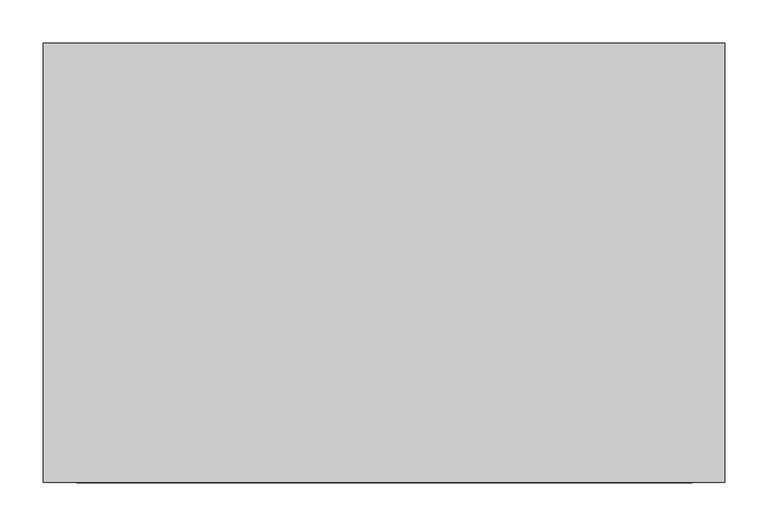
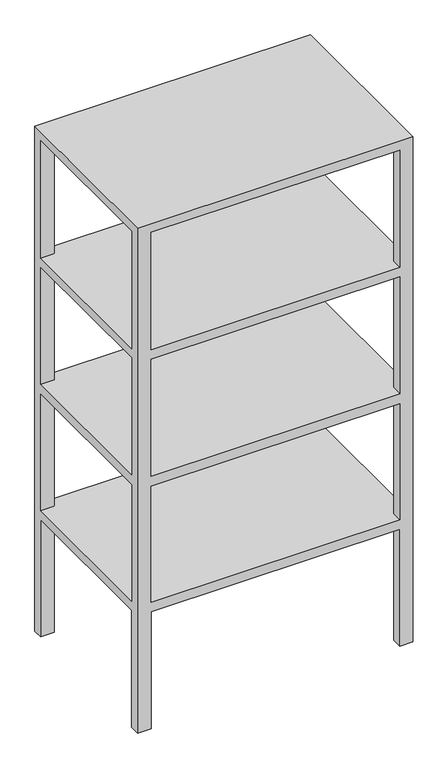
"""IFC4 building model written with IfcOpenShell, lengths in millimetres: furniture geometry, Preserved mushrrom shelf : Preserved mushrrom shelf."""

from ifc_helpers import new_model, si_unit, origin, place, context, project, spatial, faceted_brep, source, transform, mapped, element, save


def furniture_d8989670(model_context):
    return source(origin(), model_context, "Body", "Brep", [
        faceted_brep([(10489.488508, 3379.4615366, 1524.0), (9702.088508, 3379.4615366, 1524.0), (9702.088508, 2871.4615366, 1524.0), (10489.488508, 2871.4615366, 1524.0), (10489.488508, 2900.385331, 0.0), (10489.488508, 2871.4615366, 0.0), (10452.1087778, 2871.4615366, 0.0), (10452.1087778, 2900.385331, 0.0), (10489.488508, 3379.4615366, 0.0), (10489.488508, 3350.4392676, 0.0), (10452.1087778, 3350.4392676, 0.0), (10452.1087778, 3379.4615366, 0.0), (9740.9087778, 2871.4615366, 0.0), (9702.088508, 2871.4615366, 0.0), (9702.088508, 2900.385331, 0.0), (9740.9087778, 2900.385331, 0.0), (9702.088508, 3350.4392676, 0.0), (9702.088508, 3379.4615366, 0.0), (9740.9087778, 3379.4615366, 0.0), (9740.9087778, 3350.4392676, 0.0), (10452.1087778, 3379.4615366, 353.3332002), (9740.9087778, 3379.4615366, 353.3332002), (10452.1087778, 3379.4615366, 1497.6781444), (9740.9087778, 3379.4615366, 1497.6781444), (9740.9087778, 3379.4615366, 1143.0), (10452.1087778, 3379.4615366, 1143.0), (10452.1087778, 3379.4615366, 1114.8196695), (9740.9087778, 3379.4615366, 1114.8196695), (9740.9087778, 3379.4615366, 762.0), (10452.1087778, 3379.4615366, 762.0), (10452.1087778, 3379.4615366, 731.9611947), (9740.9087778, 3379.4615366, 731.9611947), (9740.9087778, 3379.4615366, 381.0), (10452.1087778, 3379.4615366, 381.0), (9702.088508, 3350.4392676, 353.3332002), (9702.088508, 2900.385331, 353.3332002), (9702.088508, 3350.8671384, 1497.6781444), (9702.088508, 2900.385331, 1497.6781444), (9702.088508, 2900.385331, 1143.0), (9702.088508, 3350.8671384, 1143.0), (9702.088508, 3350.4392676, 1114.8196695), (9702.088508, 2900.385331, 1114.8196695), (9702.088508, 2900.385331, 762.0), (9702.088508, 3350.4392676, 762.0), (9702.088508, 3350.4392676, 731.9611947), (9702.088508, 2900.385331, 731.9611947), (9702.088508, 2900.385331, 381.0), (9702.088508, 3350.4392676, 381.0), (9740.9087778, 2871.4615366, 353.3332002), (10452.1087778, 2871.4615366, 353.3332002), (9740.9087778, 2871.4615366, 1497.6781444), (10452.1087778, 2871.4615366, 1497.6781444), (10452.1087778, 2871.4615366, 1143.0), (9740.9087778, 2871.4615366, 1143.0), (9740.9087778, 2871.4615366, 1114.8196695), (10452.1087778, 2871.4615366, 1114.8196695), (10452.1087778, 2871.4615366, 762.0), (9740.9087778, 2871.4615366, 762.0), (9740.9087778, 2871.4615366, 731.9611947), (10452.1087778, 2871.4615366, 731.9611947), (10452.1087778, 2871.4615366, 381.0), (9740.9087778, 2871.4615366, 381.0), (10489.488508, 2900.385331, 353.3332002), (10489.488508, 3350.4392676, 353.3332002), (10489.488508, 2900.385331, 1497.6781444), (10489.488508, 3350.4392676, 1497.6781444), (10489.488508, 3350.4392676, 1143.0), (10489.488508, 2900.385331, 1143.0), (10489.488508, 2900.385331, 1114.8196695), (10489.488508, 3350.4392676, 1114.8196695), (10489.488508, 3350.4392676, 762.0), (10489.488508, 2900.385331, 762.0), (10489.488508, 2900.385331, 731.9611947), (10489.488508, 3350.4392676, 731.9611947), (10489.488508, 3350.4392676, 381.0), (10489.488508, 2900.385331, 381.0), (9740.9087778, 2900.385331, 1497.6781444), (9740.9087778, 3350.8671384, 1497.6781444), (10452.1087778, 3350.4392676, 1497.6781444), (10452.1087778, 2900.385331, 1497.6781444), (9740.9087778, 2900.385331, 1143.0), (10452.1087778, 2900.385331, 1143.0), (10452.1087778, 3350.4392676, 1143.0), (9740.9087778, 3350.8671384, 1143.0), (9740.9087778, 2900.385331, 1114.8196695), (9740.9087778, 3350.4392676, 1114.8196695), (10452.1087778, 3350.4392676, 1114.8196695), (10452.1087778, 2900.385331, 1114.8196695), (9740.9087778, 2900.385331, 762.0), (10452.1087778, 2900.385331, 762.0), (10452.1087778, 3350.4392676, 762.0), (9740.9087778, 3350.4392676, 762.0), (9740.9087778, 2900.385331, 731.9611947), (9740.9087778, 3350.4392676, 731.9611947), (10452.1087778, 3350.4392676, 731.9611947), (10452.1087778, 2900.385331, 731.9611947), (9740.9087778, 2900.385331, 381.0), (10452.1087778, 2900.385331, 381.0), (10452.1087778, 3350.4392676, 381.0), (9740.9087778, 3350.4392676, 381.0), (9740.9087778, 2900.385331, 353.3332002), (9740.9087778, 3350.4392676, 353.3332002), (10452.1087778, 3350.4392676, 353.3332002), (10452.1087778, 2900.385331, 353.3332002)], [[[0, 1, 2, 3]], [[4, 5, 6, 7]], [[8, 9, 10, 11]], [[12, 13, 14, 15]], [[16, 17, 18, 19]], [[1, 0, 8, 11, 20, 21, 18, 17], [22, 23, 24, 25], [26, 27, 28, 29], [30, 31, 32, 33]], [[2, 1, 17, 16, 34, 35, 14, 13], [36, 37, 38, 39], [40, 41, 42, 43], [44, 45, 46, 47]], [[3, 2, 13, 12, 48, 49, 6, 5], [50, 51, 52, 53], [54, 55, 56, 57], [58, 59, 60, 61]], [[0, 3, 5, 4, 62, 63, 9, 8], [64, 65, 66, 67], [68, 69, 70, 71], [72, 73, 74, 75]], [[76, 37, 36, 77, 23, 22, 78, 65, 64, 79, 51, 50]], [[80, 53, 52, 81, 67, 66, 82, 25, 24, 83, 39, 38]], [[76, 50, 53, 80]], [[51, 79, 81, 52]], [[79, 64, 67, 81]], [[65, 78, 82, 66]], [[78, 22, 25, 82]], [[23, 77, 83, 24]], [[77, 36, 39, 83]], [[37, 76, 80, 38]], [[84, 41, 40, 85, 27, 26, 86, 69, 68, 87, 55, 54]], [[88, 57, 56, 89, 71, 70, 90, 29, 28, 91, 43, 42]], [[84, 54, 57, 88]], [[55, 87, 89, 56]], [[87, 68, 71, 89]], [[69, 86, 90, 70]], [[86, 26, 29, 90]], [[27, 85, 91, 28]], [[85, 40, 43, 91]], [[41, 84, 88, 42]], [[92, 45, 44, 93, 31, 30, 94, 73, 72, 95, 59, 58]], [[96, 61, 60, 97, 75, 74, 98, 33, 32, 99, 47, 46]], [[92, 58, 61, 96]], [[59, 95, 97, 60]], [[95, 72, 75, 97]], [[73, 94, 98, 74]], [[94, 30, 33, 98]], [[31, 93, 99, 32]], [[93, 44, 47, 99]], [[45, 92, 96, 46]], [[100, 35, 34, 101, 21, 20, 102, 63, 62, 103, 49, 48]], [[100, 48, 12, 15]], [[49, 103, 7, 6]], [[103, 62, 4, 7]], [[63, 102, 10, 9]], [[102, 20, 11, 10]], [[21, 101, 19, 18]], [[101, 34, 16, 19]], [[35, 100, 15, 14]]]),
    ])


if __name__ == "__main__":
    model = new_model("IFC4")
    model_context = context("Model", 3, world=origin())
    ifc_project = project(units=[si_unit("LENGTHUNIT", "METRE", prefix="MILLI")], contexts=[model_context])
    site = spatial("IfcSite", under=ifc_project)
    building = spatial("IfcBuilding", under=site)
    placement = place(None, origin())
    furniture_shape = furniture_d8989670(model_context)
    element("IfcFurniture", 1, ObjectType="Preserved mushrrom shelf : Preserved mushrrom shelf", at=placement, inside=building, context=model_context, shape_type="MappedRepresentation", body=[
        mapped(furniture_shape, transform((0.0, 0.0, 0.0), x_axis=(1.0, 0.0, 0.0), y_axis=(0.0, 1.0, 0.0), z_axis=(0.0, 0.0, 1.0))),
    ])
    save(model, "model.ifc")

# Revit data of these elements
# Element 1 (IfcFurniture, "Preserved mushrrom shelf : Preserved mushrrom shelf")
#   Materials on its faces: "food"
# Materials
#   "food": class "Glass", colour RGB 233 233 233, transparency 0, Description = "Soda Lime Glass", Cost = 0
